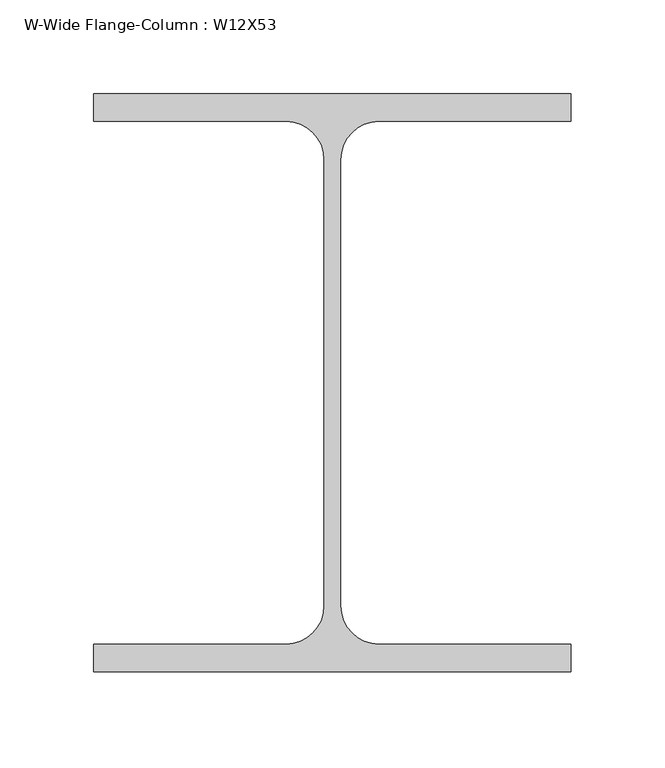
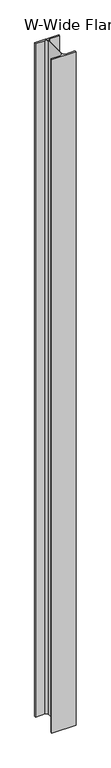
"""IFC4 building model written with IfcOpenShell, lengths in millimetres: column geometry, W-Wide Flange-Column : W12X53."""

from ifc_helpers import new_model, si_unit, point, frame, frame_2d, origin, place, context, project, spatial, polyline, circle_curve, trimmed, segment, composite_curve, outline, extrude, source, transform, mapped, element, save


def w_wide_flange_column_w12x53_fd574e43(model_context):
    return source(origin(), model_context, "Body", "SweptSolid", [
        extrude(outline(composite_curve([segment(polyline([(127.0, 153.67), (127.0, 139.065), (24.7015, 139.065)]), True, "CONTINUOUS"), segment(trimmed(circle_curve(frame_2d((24.7015, 118.745)), 20.32), [point((24.7015, 139.065))], [point((4.3815, 118.745))], True, "CARTESIAN"), True, "CONTINUOUS"), segment(polyline([(4.3815, 118.745), (4.3815, -118.745)]), True, "CONTINUOUS"), segment(trimmed(circle_curve(frame_2d((24.7015, -118.745)), 20.32), [point((4.3815, -118.745))], [point((24.7015, -139.065))], True, "CARTESIAN"), True, "CONTINUOUS"), segment(polyline([(24.7015, -139.065), (127.0, -139.065), (127.0, -153.67), (-127.0, -153.67), (-127.0, -139.065), (-24.7015, -139.065)]), True, "CONTINUOUS"), segment(trimmed(circle_curve(frame_2d((-24.7015, -118.745)), 20.32), [point((-24.7015, -139.065))], [point((-4.3815, -118.745))], True, "CARTESIAN"), True, "CONTINUOUS"), segment(polyline([(-4.3815, -118.745), (-4.3815, 118.745)]), True, "CONTINUOUS"), segment(trimmed(circle_curve(frame_2d((-24.7015, 118.745)), 20.32), [point((-4.3815, 118.745))], [point((-24.7015, 139.065))], True, "CARTESIAN"), True, "CONTINUOUS"), segment(polyline([(-24.7015, 139.065), (-127.0, 139.065), (-127.0, 153.67), (127.0, 153.67)]), True, "CONTINUOUS")], self_intersect=False)), frame((0.0, 0.0, 8756.65), z_axis=(0.0, 0.0, 1.0), x_axis=(1.0, 0.0, 0.0)), (0.0, 0.0, 1.0), 7448.55),
    ])


if __name__ == "__main__":
    model = new_model("IFC4")
    model_context = context("Model", 3, world=origin())
    ifc_project = project(units=[si_unit("LENGTHUNIT", "METRE", prefix="MILLI")], contexts=[model_context])
    site = spatial("IfcSite", under=ifc_project)
    building = spatial("IfcBuilding", under=site)
    placement = place(None, origin())
    w_wide_flange_column_w12x53_shape = w_wide_flange_column_w12x53_fd574e43(model_context)
    element("IfcColumn", 1, ObjectType="W-Wide Flange-Column : W12X53", at=placement, inside=building, context=model_context, shape_type="MappedRepresentation", body=[
        mapped(w_wide_flange_column_w12x53_shape, transform((0.0, 0.0, 0.0), x_axis=(1.0, 0.0, 0.0), y_axis=(0.0, 1.0, 0.0), z_axis=(0.0, 0.0, 1.0))),
    ])
    save(model, "model.ifc")

# Revit data of these elements
# Type "W-Wide Flange-Column : W12X53"
#   Assembly Code = "B10"
#   W = 53
#   bf = 0' - 10"
#   d = 1' - 0.1"
#   k = 0' - 1 3/8"
#   kr = 0' - 0.8"
#   tf = 0' - 0.575"
#   tw = 0' - 0.345"
#   A = 0.108333 SF
#   Structural Material [instance default] = Steel ASTM A992
# Element 1 (IfcColumn, "W-Wide Flange-Column : W12X53")
#   Materials on its faces: "Steel ASTM A992"
# Materials
#   "Steel ASTM A992": class "Metal", colour RGB 199 199 199, transparency 0, Description = "Structural steel 50ksi", Cost = 0
